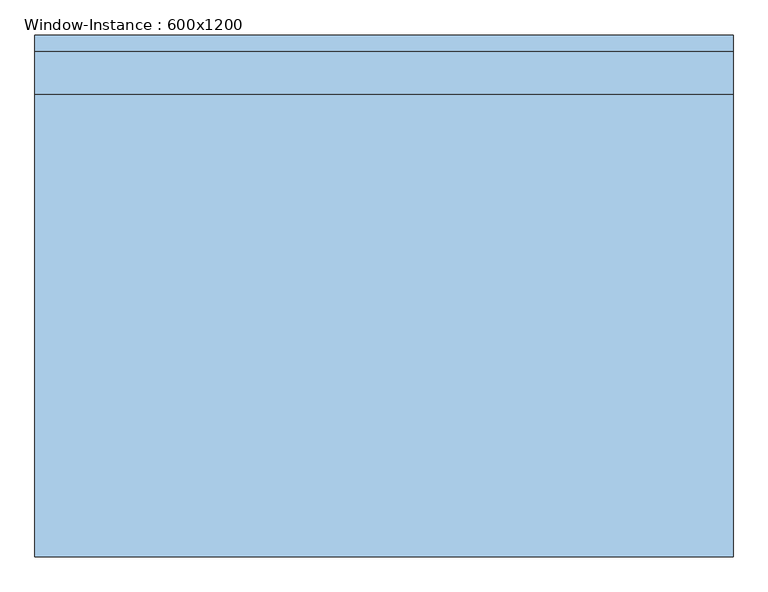
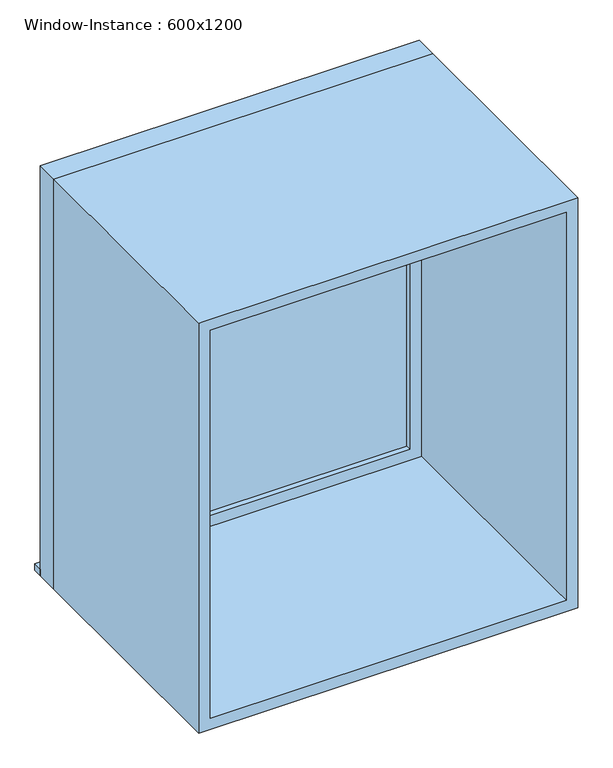
"""IFC4 building model written with IfcOpenShell, lengths in millimetres: window geometry, Window-Instance : 600x1200."""

from ifc_helpers import new_model, si_unit, frame, origin, place, context, project, spatial, polyline, outline, extrude, source, transform, mapped, element, save


def window_instance_600x1200_ad920861(model_context):
    return source(origin(), model_context, "Body", "SweptSolid", [
        extrude(outline(polyline([(-563.1, 405.4), (486.9, 405.4), (486.9, 380.0), (-563.1, 380.0), (-563.1, 405.4)])), frame((0.0, 0.0, 900.0), z_axis=(0.0, 0.0, 1.0), x_axis=(1.0, 0.0, 0.0)), (0.0, 0.0, 1.0), 19.05),
        extrude(outline(polyline([(423.4, 331.425), (-499.6, 331.425), (-499.6, 344.125), (423.4, 344.125), (423.4, 331.425)])), frame((0.0, 0.0, 963.5), z_axis=(0.0, 0.0, 1.0), x_axis=(1.0, 0.0, 0.0)), (0.0, 0.0, 1.0), 1073.0),
        extrude(outline(polyline([(2080.95, -544.05), (919.05, -544.05), (919.05, 467.85), (2080.95, 467.85), (2080.95, -544.05)]), holes=[polyline([(2036.5, -499.6), (2036.5, 423.4), (963.5, 423.4), (963.5, -499.6), (2036.5, -499.6)])]), frame((0.0, 315.55, 0.0), z_axis=(0.0, 1.0, 0.0), x_axis=(0.0, 0.0, 1.0)), (0.0, 0.0, 1.0), 44.45),
        extrude(outline(polyline([(2100.0, -563.1), (900.0, -563.1), (900.0, 486.9), (2100.0, 486.9), (2100.0, -563.1)]), holes=[polyline([(2068.25, -531.35), (2068.25, 455.15), (931.75, 455.15), (931.75, -531.35), (2068.25, -531.35)])]), frame((0.0, -380.0, 0.0), z_axis=(0.0, 1.0, 0.0), x_axis=(0.0, 0.0, 1.0)), (0.0, 0.0, 1.0), 695.55),
        extrude(outline(polyline([(2100.0, 486.9), (2100.0, -563.1), (900.0, -563.1), (900.0, 486.9), (2100.0, 486.9)]), holes=[polyline([(2080.95, 467.85), (919.05, 467.85), (919.05, -544.05), (2080.95, -544.05), (2080.95, 467.85)])]), frame((0.0, 315.55, 0.0), z_axis=(0.0, 1.0, 0.0), x_axis=(0.0, 0.0, 1.0)), (0.0, 0.0, 1.0), 64.45),
    ])


if __name__ == "__main__":
    model = new_model("IFC4")
    model_context = context("Model", 3, world=origin())
    ifc_project = project(units=[si_unit("LENGTHUNIT", "METRE", prefix="MILLI")], contexts=[model_context])
    site = spatial("IfcSite", under=ifc_project)
    building = spatial("IfcBuilding", under=site)
    placement = place(None, origin())
    window_instance_600x1200_shape = window_instance_600x1200_ad920861(model_context)
    element("IfcWindow", 1, ObjectType="Window-Instance : 600x1200", at=placement, inside=building, context=model_context, shape_type="MappedRepresentation", body=[
        mapped(window_instance_600x1200_shape, transform((0.0, 0.0, 0.0), x_axis=(1.0, 0.0, 0.0), y_axis=(0.0, 1.0, 0.0), z_axis=(0.0, 0.0, 1.0))),
    ])
    save(model, "model.ifc")

# Revit data of these elements
# Type "Window-Instance : 600x1200"
#   Type Mark = "7"
#   Construction Type Id = "GSP4R"
#   Assembly Code = "B2020100"
#   Analytic Construction = "1/8 in Pilkington single glazing"
#   Visual Light Transmittance = 0.9
#   Thermal Resistance (R) = 0.149095 (m²·K)/W
#   Solar Heat Gain Coefficient = 0.86
#   Heat Transfer Coefficient (U) = 6.70716 W/(m²·K)
#   Height [instance default] = 1200 mm
#   Default Sill Height = 900 mm
#   Width [instance default] = 600 mm
#   Window Inset = 20 mm
#   Glass Pane Material = WW-EC-GL-Storefront
#   Sash Material = WW-EC-RGB-White
#   Wall Closure = (empty or 0)
# Element 1 (IfcWindow, "Window-Instance : 600x1200")
#   Width = 1050 mm
#   Materials on its faces: "WW-EC-RGB-White", "WW-EC-GL-Storefront"
# Materials
#   "WW-EC-GL-Storefront": class "Glass", colour RGB 236 240 239, transparency 0.85, Description = "Storefront Glass", Cost = 0
#   "WW-EC-RGB-White": class "Generic", colour RGB 255 255 255, transparency 0, Comments = "If region requests off-white, swith asset color to RGB 231-228-220", Description = "Generic Color", Cost = 0
